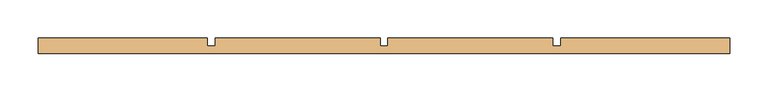
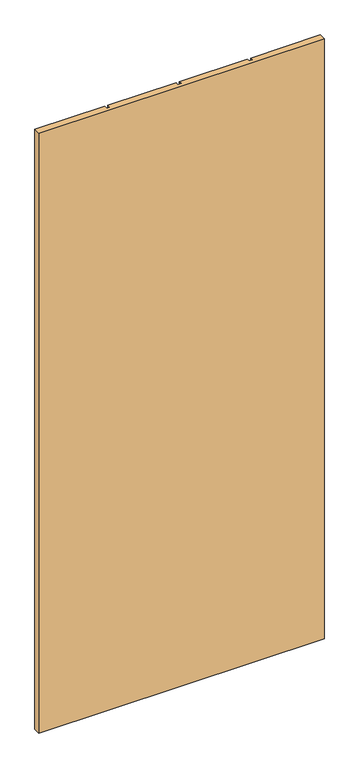
"""IFC4 building model written with IfcOpenShell, lengths in millimetres: door geometry, BA_Bi-fold door : AD_Bi-fold door - 90cm."""

from ifc_helpers import new_model, si_unit, origin, origin_with_axes, place, context, project, spatial, polyline, outline, extrude, source, transform, mapped, element, save


def door_dbf8e47a(model_context):
    return source(origin(), model_context, "Body", "SweptSolid", [
        extrude(outline(polyline([(230.0, 10.0), (450.0, 10.0), (450.0, -10.0), (-450.0, -10.0), (-450.0, 10.0), (-230.0, 10.0), (-230.0, 0.0), (-220.0, 0.0), (-220.0, 10.0), (-5.0, 10.0), (-5.0, 0.0), (5.0, 0.0), (5.0, 10.0), (220.0, 10.0), (220.0, 0.0), (230.0, 0.0), (230.0, 10.0)])), origin_with_axes(), (0.0, 0.0, 1.0), 2000.0),
    ])


if __name__ == "__main__":
    model = new_model("IFC4")
    model_context = context("Model", 3, world=origin())
    ifc_project = project(units=[si_unit("LENGTHUNIT", "METRE", prefix="MILLI")], contexts=[model_context])
    site = spatial("IfcSite", under=ifc_project)
    building = spatial("IfcBuilding", under=site)
    placement = place(None, origin())
    door_shape = door_dbf8e47a(model_context)
    element("IfcDoor", 1, ObjectType="BA_Bi-fold door : AD_Bi-fold door - 90cm", at=placement, inside=building, context=model_context, shape_type="MappedRepresentation", body=[
        mapped(door_shape, transform((0.0, 0.0, 0.0), x_axis=(1.0, 0.0, 0.0), y_axis=(0.0, 1.0, 0.0), z_axis=(0.0, 0.0, 1.0))),
    ])
    save(model, "model.ifc")

# Revit data of these elements
# Type "BA_Bi-fold door : AD_Bi-fold door - 90cm"
#   Type Mark = "49"
#   Frame Projection Ext. = 25 mm
#   Frame Projection Int. = 25 mm
#   Frame Width = 75 mm
#   Height = 2000 mm
#   Width = 900 mm
#   Define Thermal Properties by = 1
#   160cm = no
#   140cm = no
#   120cm = no
#   100cm = yes
#   Function = (empty or 0)
#   Wall Closure = (empty or 0)
# Element 1 (IfcDoor, "BA_Bi-fold door : AD_Bi-fold door - 90cm")
#   Materials on its faces: "Default"
# Materials
#   "Default": class "Generic", colour RGB 255 255 255, transparency 0, Cost = 0
